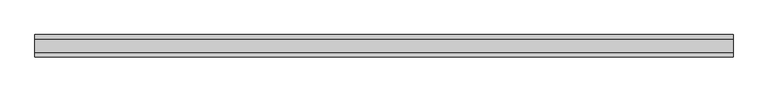
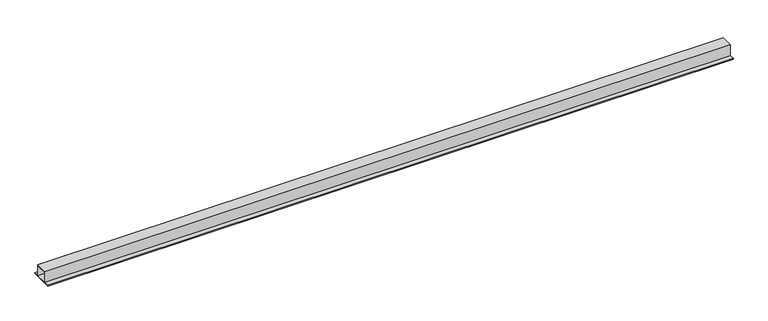
"""IFC4 building model written with IfcOpenShell, lengths in millimetres: beam geometry, NLRS_28_SF_LIB_stalen ligger THQ-AV-CWV-MMBS-SRP_gen_rsf : stalen ligger_gen__THQ_280x10-290x30-550x20."""

from ifc_helpers import new_model, si_unit, frame, origin, place, context, project, spatial, polyline, outline, extrude, source, transform, mapped, element, save


def beam_3c101ff4(model_context):
    return source(origin(), model_context, "Body", "SweptSolid", [
        extrude(outline(polyline([(143.5, 280.0), (143.5, 0.0), (263.5, 0.0), (263.5, -20.0), (-286.5, -20.0), (-286.5, 0.0), (-166.5, 0.0), (-166.5, 280.0), (143.5, 280.0)]), holes=[polyline([(133.5, 0.0), (133.5, 250.0), (-156.5, 250.0), (-156.5, 0.0), (133.5, 0.0)])]), frame((-8562.3, 0.0, 0.0), z_axis=(1.0, 0.0, 0.0), x_axis=(0.0, 1.0, 0.0)), (0.0, 0.0, 1.0), 17012.3),
    ])


if __name__ == "__main__":
    model = new_model("IFC4")
    model_context = context("Model", 3, world=origin())
    ifc_project = project(units=[si_unit("LENGTHUNIT", "METRE", prefix="MILLI")], contexts=[model_context])
    site = spatial("IfcSite", under=ifc_project)
    building = spatial("IfcBuilding", under=site)
    placement = place(None, origin())
    beam_shape = beam_3c101ff4(model_context)
    element("IfcBeam", 1, ObjectType="NLRS_28_SF_LIB_stalen ligger THQ-AV-CWV-MMBS-SRP_gen_rsf : stalen ligger_gen__THQ_280x10-290x30-550x20", at=placement, inside=building, context=model_context, shape_type="MappedRepresentation", body=[
        mapped(beam_shape, transform((0.0, 0.0, 0.0), x_axis=(1.0, 0.0, 0.0), y_axis=(0.0, 1.0, 0.0), z_axis=(0.0, 0.0, 1.0))),
    ])
    save(model, "model.ifc")

# Revit data of these elements
# Type "NLRS_28_SF_LIB_stalen ligger THQ-AV-CWV-MMBS-SRP_gen_rsf : stalen ligger_gen__THQ_280x10-290x30-550x20"
#   Type IfcGUID = "2GRbcre991teoKeCLB8MAm"
#   IfcExportAs = "IfcBeamType"
#   Type Comments = "THQ 280x10-290x30-550x20"
#   Model = " "
#   Manufacturer = " "
#   Fire Rating = " "
#   Description = "stalen ligger THQ 280x10-290x30-550x20"
#   Assembly Code = "28.11"
#   tw = 10 mm
#   tu = 20 mm
#   to = 30 mm
#   h = 280 mm
#   bu = 550 mm
#   bo = 290 mm
#   NLRS_C_lengte [instance default] = 1500 mm
#   Length [instance default] = 1500 mm
#   RSF_C_vullen_met_beton [instance default] = no
#   RSF_C_petligger = no
#   RSF_C_hoedligger = yes
#   Structural Material = NLRS_h2_staal_gen_rsf
#   Keynote = ""
# Element 1 (IfcBeam, "NLRS_28_SF_LIB_stalen ligger THQ-AV-CWV-MMBS-SRP_gen_rsf : stalen ligger_gen__THQ_280x10-290x30-550x20")
#   NLRS_C_lengte = 16900 mm
#   Materials on its faces: "NLRS_h2_staal_gen_rsf"
# Materials
#   "NLRS_h2_staal_gen_rsf": class "H - Metaal", colour RGB 189 187 185, transparency 0, Keynote = "h2", Manufacturer = "Revit Standards Foundation", URL = "www.revitstandards.org", Description = "staal", Cost = 0
